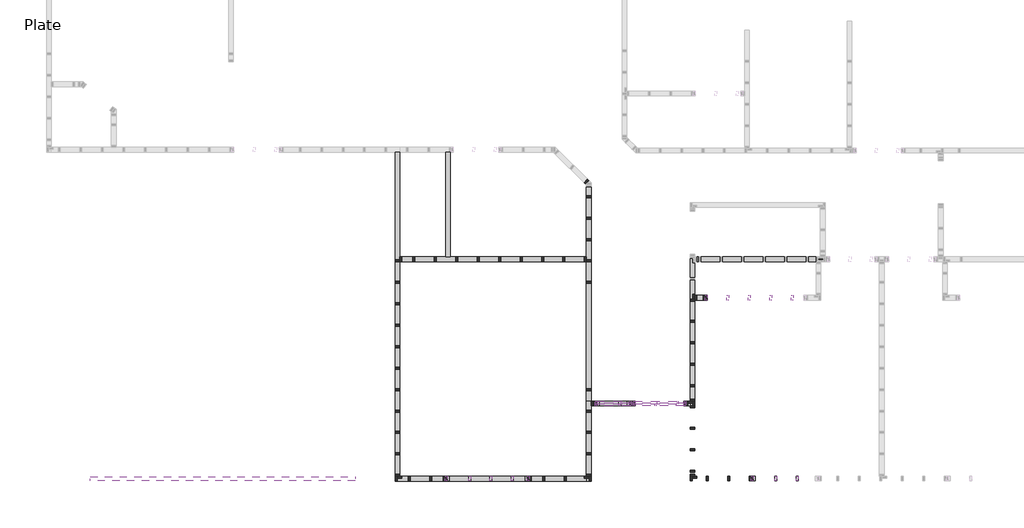
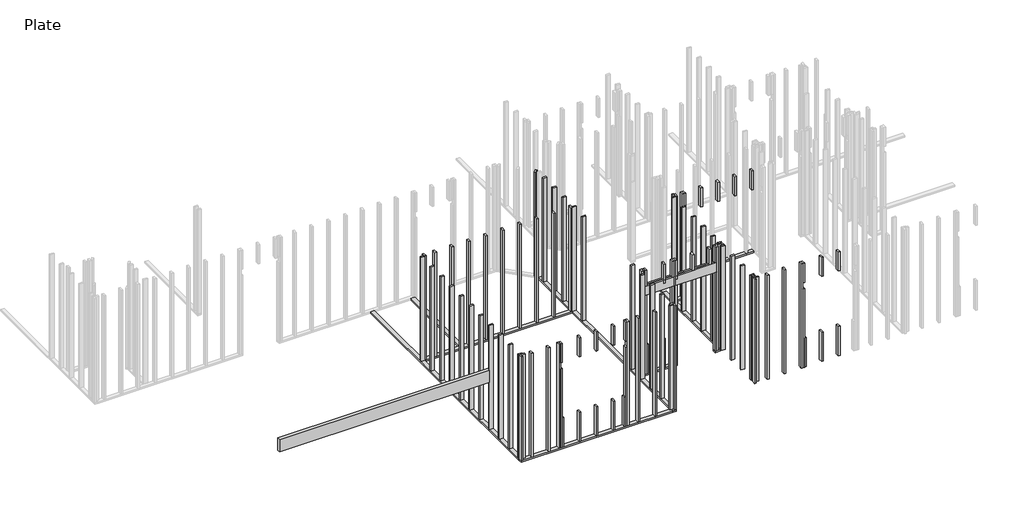
# One storey, part 1 of 5: 106 columns, 16 beams.
"""IFC4 building model written with IfcOpenShell, lengths in millimetres."""

import ifcopenshell
import ifcopenshell.guid

model = None  # the IFC model being written
_history = None  # IfcOwnerHistory: only IFC2X3 demands one
_inside = {}  # id of a spatial element -> (the spatial element, [elements in it])
_under = {}  # id of a project, library or spatial element -> (it, [spatial elements below it])
_declared = {}  # id of a project -> (the project, [libraries it declares])
_typed = {}  # id of a type object -> (the type object, [elements of that type])
_made_of = {}  # id of a material, layer set ... -> (it, [elements and type objects made of it])


def new_model(schema):
    """Start an empty IFC model of exactly this schema.

    Asked for "IFC4X3", IfcOpenShell would pick the latest addendum, in which some entities
    have other attributes; the version numbers below select the first issue.
    IFC2X3 requires an IfcOwnerHistory on every rooted entity: one is made here for all.
    """
    global model, _history
    if schema == "IFC4X3":
        model = ifcopenshell.file(schema_version=(4, 3, 0, 0))
    else:
        model = ifcopenshell.file(schema=schema)
    _inside.clear()
    _under.clear()
    _declared.clear()
    _typed.clear()
    _made_of.clear()
    _history = None
    if model.schema == "IFC2X3":
        org = make("IfcOrganization", Name="unknown")
        user = make(
            "IfcPersonAndOrganization",
            ThePerson=make("IfcPerson", FamilyName="unknown"),
            TheOrganization=org,
        )
        app = make(
            "IfcApplication",
            ApplicationDeveloper=org,
            Version="unknown",
            ApplicationFullName="unknown",
            ApplicationIdentifier="unknown",
        )
        _history = make(
            "IfcOwnerHistory",
            OwningUser=user,
            OwningApplication=app,
            ChangeAction="ADDED",
            CreationDate=0,
        )
    return model


def make(cls, **values):
    """One entity of the class cls with the attributes given. An attribute that is None is left unset."""
    return model.create_entity(
        cls, **{name: value for name, value in values.items() if value is not None}
    )


def rooted(cls, **values):
    """An entity with a GlobalId (a new one), such as an element, a storey or a relation."""
    return make(cls, GlobalId=ifcopenshell.guid.new(), OwnerHistory=_history, **values)


def si_unit(unit_type, name, prefix=None):
    """IfcSIUnit, for example si_unit("LENGTHUNIT", "METRE", prefix="MILLI")."""
    return make("IfcSIUnit", UnitType=unit_type, Prefix=prefix, Name=name)


def assignment(units):
    """IfcUnitAssignment: the units of a project."""
    return None if units is None else make("IfcUnitAssignment", Units=units)


def point(xyz):
    """IfcCartesianPoint."""
    return None if xyz is None else make("IfcCartesianPoint", Coordinates=xyz)


def direction(xyz):
    """IfcDirection."""
    return None if xyz is None else make("IfcDirection", DirectionRatios=xyz)


def frame(location, z_axis=None, x_axis=None):
    """IfcAxis2Placement3D, a coordinate frame: its origin and axes. An axis left out is left unset."""
    return make(
        "IfcAxis2Placement3D",
        Location=point(location),
        Axis=direction(z_axis),
        RefDirection=direction(x_axis),
    )


def origin():
    """The frame at (0, 0, 0) with its axes left unset."""
    return frame((0.0, 0.0, 0.0))


def place(relative_to, where):
    """IfcLocalPlacement: puts the frame where relative to a parent placement (None: the world)."""
    return make(
        "IfcLocalPlacement", PlacementRelTo=relative_to, RelativePlacement=where
    )


def context(
    kind, dimensions, precision=None, world=None, true_north=None, identifier=None
):
    """IfcGeometricRepresentationContext, for example the 3D "Model" context."""
    return make(
        "IfcGeometricRepresentationContext",
        ContextIdentifier=identifier,
        ContextType=kind,
        CoordinateSpaceDimension=dimensions,
        Precision=precision,
        WorldCoordinateSystem=world,
        TrueNorth=true_north,
    )


def project(units=None, contexts=None):
    """IfcProject with its units and contexts."""
    return rooted(
        "IfcProject",
        Name="project",
        RepresentationContexts=contexts,
        UnitsInContext=assignment(units),
    )


def spatial(cls, under=None, at=None, **own):
    """A site, building, storey or space (cls), placed at a placement, below another one or the project."""
    s = rooted(cls, ObjectPlacement=at, **own)
    if under is not None:
        _under.setdefault(under.id(), (under, []))[1].append(s)
    return s


def polyline(points):
    """IfcPolyline through the points."""
    return make("IfcPolyline", Points=[point(p) for p in points])


def outline(outer, holes=None, kind="AREA"):
    """IfcArbitraryClosedProfileDef: a profile drawn as a closed curve; with holes, ...WithVoids."""
    if holes is None:
        return make("IfcArbitraryClosedProfileDef", ProfileType=kind, OuterCurve=outer)
    return make(
        "IfcArbitraryProfileDefWithVoids",
        ProfileType=kind,
        OuterCurve=outer,
        InnerCurves=holes,
    )


def extrude(swept, where, along, depth):
    """IfcExtrudedAreaSolid: the profile swept, set in the frame where, extruded along a direction by depth."""
    return make(
        "IfcExtrudedAreaSolid",
        SweptArea=swept,
        Position=where,
        ExtrudedDirection=direction(along),
        Depth=depth,
    )


def shape(context_of_items, identifier, shape_type, items):
    """IfcShapeRepresentation: the items that make up one representation, for example the "Body"."""
    return make(
        "IfcShapeRepresentation",
        ContextOfItems=context_of_items,
        RepresentationIdentifier=identifier,
        RepresentationType=shape_type,
        Items=items,
    )


def source(mapping_origin, context_of_items, identifier, shape_type, items):
    """IfcRepresentationMap: a shape defined once, which mapped items show again and again."""
    return make(
        "IfcRepresentationMap",
        MappingOrigin=mapping_origin,
        MappedRepresentation=shape(context_of_items, identifier, shape_type, items),
    )


def transform(
    local_origin,
    x_axis=None,
    y_axis=None,
    z_axis=None,
    scale=None,
    scale2=None,
    scale3=None,
    uniform=True,
):
    """IfcCartesianTransformationOperator3D, or its non-uniform kind. x_axis, y_axis, z_axis: its Axis1, 2, 3."""
    if uniform:
        return make(
            "IfcCartesianTransformationOperator3D",
            Axis1=direction(x_axis),
            Axis2=direction(y_axis),
            LocalOrigin=point(local_origin),
            Scale=scale,
            Axis3=direction(z_axis),
        )
    return make(
        "IfcCartesianTransformationOperator3DnonUniform",
        Axis1=direction(x_axis),
        Axis2=direction(y_axis),
        LocalOrigin=point(local_origin),
        Scale=scale,
        Axis3=direction(z_axis),
        Scale2=scale2,
        Scale3=scale3,
    )


def mapped(mapping_source, mapping_target):
    """IfcMappedItem: shows the shape of a source again, moved by a transform."""
    return make(
        "IfcMappedItem", MappingSource=mapping_source, MappingTarget=mapping_target
    )


def made_of(thing, what):
    """Note that an element or type object is made of a material, layer set ...; save() writes the relation."""
    if what is not None:
        _made_of.setdefault(what.id(), (what, []))[1].append(thing)
    return thing


def element(
    cls,
    number,
    at=None,
    inside=None,
    cuts=None,
    type_object=None,
    material=None,
    context=None,
    identifier="Body",
    shape_type=None,
    held_by="IfcProductDefinitionShape",
    body=None,
    shapes=None,
    **own,
):
    """One element of the class cls, such as IfcWall. Its Tag is "e" and its number.

    at: its placement. inside: the storey or other place that contains it. cuts: it is an
    opening in that element (IfcRelVoidsElement). A single representation is given by context,
    identifier, shape_type and body (its items); several are given by shapes. held_by: the class
    of the entity that holds the representations. save() writes the other relations.
    """
    e = rooted(cls, Tag="e%d" % number, ObjectPlacement=at, **own)
    if body is not None:
        shapes = [shape(context, identifier, shape_type, body)]
    if shapes is not None:
        e.Representation = make(held_by, Representations=shapes)
    if inside is not None:
        _inside.setdefault(inside.id(), (inside, []))[1].append(e)
    if cuts is not None:
        rooted(
            "IfcRelVoidsElement", RelatingBuildingElement=cuts, RelatedOpeningElement=e
        )
    if type_object is not None:
        _typed.setdefault(type_object.id(), (type_object, []))[1].append(e)
    return made_of(e, material)


def aggregate(whole, parts):
    """IfcRelAggregates: a whole, such as a stair, and the parts it consists of."""
    return rooted("IfcRelAggregates", RelatingObject=whole, RelatedObjects=parts)


def save(model, path):
    """Write the relations noted so far, then the file.

    IfcRelAggregates (storeys below a building ...), IfcRelContainedInSpatialStructure (elements
    in a storey), IfcRelDefinesByType, IfcRelAssociatesMaterial and IfcRelDeclares: one each for
    every whole, place, type object, material and project.
    """
    for whole, parts in _under.values():
        aggregate(whole, parts)
    for where, things in _inside.values():
        rooted(
            "IfcRelContainedInSpatialStructure",
            RelatedElements=things,
            RelatingStructure=where,
        )
    for kind, things in _typed.values():
        rooted("IfcRelDefinesByType", RelatedObjects=things, RelatingType=kind)
    for what, things in _made_of.values():
        rooted("IfcRelAssociatesMaterial", RelatedObjects=things, RelatingMaterial=what)
    for by, libraries in _declared.values():
        rooted("IfcRelDeclares", RelatingContext=by, RelatedDefinitions=libraries)
    model.write(path)


def dimension_lumber_2x10_header_exterior_0c196d91(model_context):
    return source(origin(), model_context, "Body", "SweptSolid", [
        extrude(outline(polyline([(468.709375, 19.05), (468.709375, -19.05), (-217.090625, -19.05), (-217.090625, 19.05), (468.709375, 19.05)])), frame((0.0, 0.0, -117.475), z_axis=(0.0, 0.0, 1.0), x_axis=(1.0, 0.0, 0.0)), (0.0, 0.0, 1.0), 234.95),
    ])


def dimension_lumber_2x10_header_exterior_3e47137c(model_context):
    return source(origin(), model_context, "Body", "SweptSolid", [
        extrude(outline(polyline([(468.709375, 19.05), (468.709375, -19.05), (-521.890625, -19.05), (-521.890625, 19.05), (468.709375, 19.05)])), frame((0.0, 0.0, -117.475), z_axis=(0.0, 0.0, 1.0), x_axis=(1.0, 0.0, 0.0)), (0.0, 0.0, 1.0), 234.95),
    ])


def dimension_lumber_supporting_bottom_plate_a3b44643(model_context):
    return source(origin(), model_context, "Body", "SweptSolid", [
        extrude(outline(polyline([(84.225, 44.45), (84.225, -44.45), (-39.775, -44.45), (-39.775, 44.45), (84.225, 44.45)])), frame((0.0, 0.0, -19.05), z_axis=(0.0, 0.0, 1.0), x_axis=(1.0, 0.0, 0.0)), (0.0, 0.0, 1.0), 38.1),
    ])


def dimension_lumber_supporting_bottom_plate_5d1fa65a(model_context):
    return source(origin(), model_context, "Body", "SweptSolid", [
        extrude(outline(polyline([(755.65, 44.45), (755.65, -44.45), (-755.65, -44.45), (-755.65, 44.45), (755.65, 44.45)])), frame((0.0, 0.0, -19.05), z_axis=(0.0, 0.0, 1.0), x_axis=(1.0, 0.0, 0.0)), (0.0, 0.0, 1.0), 38.1),
    ])


def dimension_lumber_supporting_bottom_plate_2403c2db(model_context):
    return source(origin(), model_context, "Body", "SweptSolid", [
        extrude(outline(polyline([(1858.9625, 44.45), (1858.9625, -44.45), (-1770.0625, -44.45), (-1770.0625, 44.45), (1858.9625, 44.45)])), frame((0.0, 0.0, -19.05), z_axis=(0.0, 0.0, 1.0), x_axis=(1.0, 0.0, 0.0)), (0.0, 0.0, 1.0), 38.1),
    ])


def dimension_lumber_supporting_bottom_plate_8d258b52(model_context):
    return source(origin(), model_context, "Body", "SweptSolid", [
        extrude(outline(polyline([(3074.9875, 44.45), (3074.9875, -44.45), (-3074.9875, -44.45), (-3074.9875, 44.45), (3074.9875, 44.45)])), frame((0.0, 0.0, -19.05), z_axis=(0.0, 0.0, 1.0), x_axis=(1.0, 0.0, 0.0)), (0.0, 0.0, 1.0), 38.1),
    ])


def dimension_lumber_supporting_bottom_plate_bb9f9100(model_context):
    return source(origin(), model_context, "Body", "SweptSolid", [
        extrude(outline(polyline([(995.3625, 44.45), (995.3625, -44.45), (-995.3625, -44.45), (-995.3625, 44.45), (995.3625, 44.45)])), frame((0.0, 0.0, -19.05), z_axis=(0.0, 0.0, 1.0), x_axis=(1.0, 0.0, 0.0)), (0.0, 0.0, 1.0), 38.1),
    ])


def dimension_lumber_supporting_bottom_plate_9bff56d6(model_context):
    return source(origin(), model_context, "Body", "SweptSolid", [
        extrude(outline(polyline([(-1544.0421875, 44.45), (-1544.0421875, -44.45), (-4097.9328125, -44.45), (-4097.9328125, 44.45), (-1544.0421875, 44.45)])), frame((0.0, 0.0, -19.05), z_axis=(0.0, 0.0, 1.0), x_axis=(1.0, 0.0, 0.0)), (0.0, 0.0, 1.0), 38.1),
    ])


def dimension_lumber_supporting_bottom_plate_2ddee0ef(model_context):
    return source(origin(), model_context, "Body", "SweptSolid", [
        extrude(outline(polyline([(1771.65, 44.45), (1771.65, -44.45), (-1768.475, -44.45), (-1768.475, 44.45), (1771.65, 44.45)])), frame((0.0, 0.0, -19.05), z_axis=(0.0, 0.0, 1.0), x_axis=(1.0, 0.0, 0.0)), (0.0, 0.0, 1.0), 38.1),
    ])


def dimension_lumber_supporting_bottom_plate_736f332d(model_context):
    return source(origin(), model_context, "Body", "SweptSolid", [
        extrude(outline(polyline([(139.7000003, 44.45), (139.7000003, -44.45), (-95.2500003, -44.45), (-95.2500003, 44.45), (139.7000003, 44.45)])), frame((0.0, 0.0, -19.05), z_axis=(0.0, 0.0, 1.0), x_axis=(1.0, 0.0, 0.0)), (0.0, 0.0, 1.0), 38.1),
    ])


def dimension_lumber_supporting_bottom_plate_ae810c3f(model_context):
    return source(origin(), model_context, "Body", "SweptSolid", [
        extrude(outline(polyline([(1404.540625, 44.45), (1404.540625, -44.45), (-1385.490625, -44.45), (-1385.490625, 44.45), (1404.540625, 44.45)])), frame((0.0, 0.0, -19.05), z_axis=(0.0, 0.0, 1.0), x_axis=(1.0, 0.0, 0.0)), (0.0, 0.0, 1.0), 38.1),
    ])


def dimension_lumber_supporting_bottom_plate_d3939b75(model_context):
    return source(origin(), model_context, "Body", "SweptSolid", [
        extrude(outline(polyline([(398.375, 44.45), (398.375, -44.45), (-442.825, -44.45), (-442.825, 44.45), (398.375, 44.45)])), frame((0.0, 0.0, -19.05), z_axis=(0.0, 0.0, 1.0), x_axis=(1.0, 0.0, 0.0)), (0.0, 0.0, 1.0), 38.1),
    ])


def glulam_western_species_20871a06(model_context):
    return source(origin(), model_context, "Body", "SweptSolid", [
        extrude(outline(polyline([(481.409375, 39.6875), (481.409375, -39.6875), (-4547.790625, -39.6875), (-4547.790625, 39.6875), (481.409375, 39.6875)])), frame((0.0, 0.0, -152.4), z_axis=(0.0, 0.0, 1.0), x_axis=(1.0, 0.0, 0.0)), (0.0, 0.0, 1.0), 304.8),
    ])


def dimension_lumber_column_2x4_07183c39(model_context):
    return source(origin(), model_context, "Body", "SweptSolid", [
        extrude(outline(polyline([(19.05, 44.45), (19.05, -44.45), (-19.05, -44.45), (-19.05, 44.45), (19.05, 44.45)])), frame((0.0, 0.0, 56.35625), z_axis=(0.0, 0.0, 1.0), x_axis=(1.0, 0.0, 0.0)), (0.0, 0.0, 1.0), 2636.04375),
    ])


def dimension_lumber_column_2x4_f24b5bbb(model_context):
    return source(origin(), model_context, "Body", "SweptSolid", [
        extrude(outline(polyline([(19.05, -44.45), (-19.05, -44.45), (-19.05, 44.45), (19.05, 44.45), (19.05, -44.45)])), frame((0.0, 0.0, 56.35625), z_axis=(0.0, 0.0, 1.0), x_axis=(1.0, 0.0, 0.0)), (0.0, 0.0, 1.0), 2636.04375),
    ])


def dimension_lumber_column_2x4_0f816ddf(model_context):
    return source(origin(), model_context, "Body", "SweptSolid", [
        extrude(outline(polyline([(19.05, 44.45), (19.05, -44.45), (-19.05, -44.45), (-19.05, 44.45), (19.05, 44.45)])), frame((0.0, 0.0, 56.35625), z_axis=(0.0, 0.0, 1.0), x_axis=(1.0, 0.0, 0.0)), (0.0, 0.0, 1.0), 1999.853125),
    ])


def dimension_lumber_column_2x4_c2f848da(model_context):
    return source(origin(), model_context, "Body", "SweptSolid", [
        extrude(outline(polyline([(19.05, 44.45), (19.05, -44.45), (-19.05, -44.45), (-19.05, 44.45), (19.05, 44.45)])), frame((0.0, 0.0, 2208.609375), z_axis=(0.0, 0.0, 1.0), x_axis=(1.0, 0.0, 0.0)), (0.0, 0.0, 1.0), 483.790625),
    ])


def dimension_lumber_column_2x4_35883525(model_context):
    return source(origin(), model_context, "Body", "SweptSolid", [
        extrude(outline(polyline([(19.05, 44.45), (19.05, -44.45), (-19.05, -44.45), (-19.05, 44.45), (19.05, 44.45)])), frame((0.0, 0.0, 56.35625), z_axis=(0.0, 0.0, 1.0), x_axis=(1.0, 0.0, 0.0)), (0.0, 0.0, 1.0), 742.553125),
    ])


model = new_model("IFC4")

# Units and contexts
model_context = context("Model", 3, world=origin())
ifc_project = project(units=[si_unit("LENGTHUNIT", "METRE", prefix="MILLI")], contexts=[model_context])

# Site, building, storey
site = spatial("IfcSite", under=ifc_project)
building = spatial("IfcBuilding", under=site)
storey = spatial("IfcBuildingStorey", under=building, Name="Plate", Elevation=56.35625)

# Beams
placement = place(None, origin())
dimension_lumber_2x10_header_exterior_shape = dimension_lumber_2x10_header_exterior_0c196d91(model_context)
element("IfcBeam", 1, ObjectType="Dimension Lumber : 2x10 Header Exterior", at=placement, inside=storey, context=model_context, shape_type="MappedRepresentation", body=[
    mapped(dimension_lumber_2x10_header_exterior_shape, transform((4633.6941499, -4308.1040947, 2173.684375), x_axis=(-1.0, 0.0, 0.0), y_axis=(0.0, -1.0, 0.0), z_axis=(0.0, 0.0, 1.0))),
])
dimension_lumber_2x10_header_exterior_2_shape = dimension_lumber_2x10_header_exterior_3e47137c(model_context)
element("IfcBeam", 2, ObjectType="Dimension Lumber : 2x10 Header Exterior", at=placement, inside=storey, context=model_context, shape_type="MappedRepresentation", body=[
    mapped(dimension_lumber_2x10_header_exterior_2_shape, transform((5357.5941499, -4308.1040947, 2173.684375), x_axis=(-1.0, 0.0, 0.0), y_axis=(0.0, -1.0, 0.0), z_axis=(0.0, 0.0, 1.0))),
])
element("IfcBeam", 3, ObjectType="Dimension Lumber : 2x10 Header Interior", at=placement, inside=storey, context=model_context, shape_type="MappedRepresentation", body=[
    mapped(dimension_lumber_2x10_header_exterior_shape, transform((4633.6941499, -4257.3040947, 2173.684375), x_axis=(-1.0, 0.0, 0.0), y_axis=(0.0, -1.0, 0.0), z_axis=(0.0, 0.0, 1.0))),
])
element("IfcBeam", 4, ObjectType="Dimension Lumber : 2x10 Header Interior", at=placement, inside=storey, context=model_context, shape_type="MappedRepresentation", body=[
    mapped(dimension_lumber_2x10_header_exterior_2_shape, transform((5357.5941499, -4257.3040947, 2173.684375), x_axis=(-1.0, 0.0, 0.0), y_axis=(0.0, -1.0, 0.0), z_axis=(0.0, 0.0, 1.0))),
])
element("IfcBeam", 5, ObjectType="Dimension Lumber : Supporting Bottom Plate", at=placement, inside=storey, context=model_context, shape_type="SweptSolid", body=[
    extrude(outline(polyline([(4085.7847749, -4238.2540947), (3996.8847749, -4238.2540947), (3996.8847749, -134.8776804), (4085.7847749, -98.0540947), (4085.7847749, -4238.2540947)])), frame((0.0, 0.0, 18.25625), z_axis=(0.0, 0.0, 1.0), x_axis=(1.0, 0.0, 0.0)), (0.0, 0.0, 1.0), 38.1),
])
dimension_lumber_supporting_bottom_plate_shape = dimension_lumber_supporting_bottom_plate_a3b44643(model_context)
element("IfcBeam", 6, ObjectType="Dimension Lumber : Supporting Bottom Plate", at=placement, inside=storey, context=model_context, shape_type="MappedRepresentation", body=[
    mapped(dimension_lumber_supporting_bottom_plate_shape, transform((5925.6097749, -4282.7040947, 37.30625), x_axis=(-1.0, 0.0, 0.0), y_axis=(0.0, -1.0, 0.0), z_axis=(0.0, 0.0, 1.0))),
])
dimension_lumber_supporting_bottom_plate_2_shape = dimension_lumber_supporting_bottom_plate_5d1fa65a(model_context)
element("IfcBeam", 7, ObjectType="Dimension Lumber : Supporting Bottom Plate", at=placement, inside=storey, context=model_context, shape_type="MappedRepresentation", body=[
    mapped(dimension_lumber_supporting_bottom_plate_2_shape, transform((4041.3347749, -4993.9040947, 37.30625), x_axis=(0.0, -1.0, 0.0), y_axis=(1.0, 0.0, 0.0), z_axis=(0.0, 0.0, 1.0))),
])
dimension_lumber_supporting_bottom_plate_3_shape = dimension_lumber_supporting_bottom_plate_2403c2db(model_context)
element("IfcBeam", 8, ObjectType="Dimension Lumber : Supporting Bottom Plate", at=placement, inside=storey, context=model_context, shape_type="MappedRepresentation", body=[
    mapped(dimension_lumber_supporting_bottom_plate_3_shape, transform((2226.8222749, -5705.1040947, 37.30625), x_axis=(-1.0, 0.0, 0.0), y_axis=(0.0, -1.0, 0.0), z_axis=(0.0, 0.0, 1.0))),
])
dimension_lumber_supporting_bottom_plate_4_shape = dimension_lumber_supporting_bottom_plate_8d258b52(model_context)
element("IfcBeam", 9, ObjectType="Dimension Lumber : Supporting Bottom Plate", at=placement, inside=storey, context=model_context, shape_type="MappedRepresentation", body=[
    mapped(dimension_lumber_supporting_bottom_plate_4_shape, transform((412.3097749, -2585.6665947, 37.30625), x_axis=(0.0, 1.0, 0.0), y_axis=(-1.0, 0.0, 0.0), z_axis=(0.0, 0.0, 1.0))),
])
dimension_lumber_supporting_bottom_plate_5_shape = dimension_lumber_supporting_bottom_plate_bb9f9100(model_context)
element("IfcBeam", 10, ObjectType="Dimension Lumber : Supporting Bottom Plate", at=placement, inside=storey, context=model_context, shape_type="MappedRepresentation", body=[
    mapped(dimension_lumber_supporting_bottom_plate_5_shape, transform((1374.3347749, -506.0415947, 37.30625), x_axis=(0.0, -1.0, 0.0), y_axis=(1.0, 0.0, 0.0), z_axis=(0.0, 0.0, 1.0))),
])
dimension_lumber_supporting_bottom_plate_6_shape = dimension_lumber_supporting_bottom_plate_9bff56d6(model_context)
element("IfcBeam", 11, ObjectType="Dimension Lumber : Supporting Bottom Plate", at=placement, inside=storey, context=model_context, shape_type="MappedRepresentation", body=[
    mapped(dimension_lumber_supporting_bottom_plate_6_shape, transform((4510.2425874, -1545.8540947, 37.30625), x_axis=(-1.0, 0.0, 0.0), y_axis=(0.0, -1.0, 0.0), z_axis=(0.0, 0.0, 1.0))),
])
dimension_lumber_supporting_bottom_plate_7_shape = dimension_lumber_supporting_bottom_plate_2ddee0ef(model_context)
element("IfcBeam", 12, ObjectType="Dimension Lumber : Supporting Bottom Plate", at=placement, inside=storey, context=model_context, shape_type="MappedRepresentation", body=[
    mapped(dimension_lumber_supporting_bottom_plate_7_shape, transform((2225.2347749, -1545.8540947, 37.30625), x_axis=(1.0, 0.0, 0.0), y_axis=(0.0, 1.0, 0.0), z_axis=(0.0, 0.0, 1.0))),
])
dimension_lumber_supporting_bottom_plate_8_shape = dimension_lumber_supporting_bottom_plate_736f332d(model_context)
element("IfcBeam", 13, ObjectType="Dimension Lumber : Supporting Bottom Plate", at=placement, inside=storey, context=model_context, shape_type="MappedRepresentation", body=[
    mapped(dimension_lumber_supporting_bottom_plate_8_shape, transform((6149.5347752, -2276.1040947, 37.30625), x_axis=(1.0, 0.0, 0.0), y_axis=(0.0, 1.0, 0.0), z_axis=(0.0, 0.0, 1.0))),
])
dimension_lumber_supporting_bottom_plate_9_shape = dimension_lumber_supporting_bottom_plate_ae810c3f(model_context)
element("IfcBeam", 14, ObjectType="Dimension Lumber : Supporting Bottom Plate", at=placement, inside=storey, context=model_context, shape_type="MappedRepresentation", body=[
    mapped(dimension_lumber_supporting_bottom_plate_9_shape, transform((6009.8347749, -2833.7134697, 37.30625), x_axis=(0.0, -1.0, 0.0), y_axis=(1.0, 0.0, 0.0), z_axis=(0.0, 0.0, 1.0))),
])
dimension_lumber_supporting_bottom_plate_10_shape = dimension_lumber_supporting_bottom_plate_d3939b75(model_context)
element("IfcBeam", 15, ObjectType="Dimension Lumber : Supporting Bottom Plate", at=placement, inside=storey, context=model_context, shape_type="MappedRepresentation", body=[
    mapped(dimension_lumber_supporting_bottom_plate_10_shape, transform((4484.1597749, -4282.7040947, 37.30625), x_axis=(-1.0, 0.0, 0.0), y_axis=(0.0, -1.0, 0.0), z_axis=(0.0, 0.0, 1.0))),
])
glulam_western_species_shape = glulam_western_species_20871a06(model_context)
element("IfcBeam", 16, ObjectType="Glulam-Western Species : 3.125x12 Headers Exterior", at=placement, inside=storey, context=model_context, shape_type="MappedRepresentation", body=[
    mapped(glulam_western_species_shape, transform((-4932.4058501, -5705.1040947, 2457.45), x_axis=(-1.0, 0.0, 0.0), y_axis=(0.0, -1.0, 0.0), z_axis=(0.0, 0.0, 1.0))),
])

# Columns
dimension_lumber_column_2x4_shape = dimension_lumber_column_2x4_07183c39(model_context)
element("IfcColumn", 17, ObjectType="Dimension Lumber-Column : 2x4", at=placement, inside=storey, context=model_context, shape_type="MappedRepresentation", body=[
    mapped(dimension_lumber_column_2x4_shape, transform((6695.6347755, -5705.1040947, 0.0), x_axis=(1.0, 0.0, 0.0), y_axis=(0.0, 1.0, 0.0), z_axis=(0.0, 0.0, 1.0))),
])
element("IfcColumn", 18, ObjectType="Dimension Lumber-Column : 2x4", at=placement, inside=storey, context=model_context, shape_type="MappedRepresentation", body=[
    mapped(dimension_lumber_column_2x4_shape, transform((6289.2347755, -5705.1040947, 0.0), x_axis=(1.0, 0.0, 0.0), y_axis=(0.0, 1.0, 0.0), z_axis=(0.0, 0.0, 1.0))),
])
element("IfcColumn", 19, ObjectType="Dimension Lumber-Column : 2x4", at=placement, inside=storey, context=model_context, shape_type="MappedRepresentation", body=[
    mapped(dimension_lumber_column_2x4_shape, transform((5984.4347749, -5705.1040947, 0.0), x_axis=(1.0, 0.0, 0.0), y_axis=(0.0, 1.0, 0.0), z_axis=(0.0, 0.0, 1.0))),
])
element("IfcColumn", 20, ObjectType="Dimension Lumber-Column : 2x4", at=placement, inside=storey, context=model_context, shape_type="MappedRepresentation", body=[
    mapped(dimension_lumber_column_2x4_shape, transform((3596.8347749, -5705.1040947, 0.0), x_axis=(1.0, 0.0, 0.0), y_axis=(0.0, 1.0, 0.0), z_axis=(0.0, 0.0, 1.0))),
])
element("IfcColumn", 21, ObjectType="Dimension Lumber-Column : 2x4", at=placement, inside=storey, context=model_context, shape_type="MappedRepresentation", body=[
    mapped(dimension_lumber_column_2x4_shape, transform((3190.4347749, -5705.1040947, 0.0), x_axis=(1.0, 0.0, 0.0), y_axis=(0.0, 1.0, 0.0), z_axis=(0.0, 0.0, 1.0))),
])
element("IfcColumn", 22, ObjectType="Dimension Lumber-Column : 2x4", at=placement, inside=storey, context=model_context, shape_type="MappedRepresentation", body=[
    mapped(dimension_lumber_column_2x4_shape, transform((2936.4347749, -5705.1040947, 0.0), x_axis=(1.0, 0.0, 0.0), y_axis=(0.0, 1.0, 0.0), z_axis=(0.0, 0.0, 1.0))),
])
element("IfcColumn", 23, ObjectType="Dimension Lumber-Column : 2x4", at=placement, inside=storey, context=model_context, shape_type="MappedRepresentation", body=[
    mapped(dimension_lumber_column_2x4_shape, transform((1298.1347743, -5705.1040947, 0.0), x_axis=(1.0, 0.0, 0.0), y_axis=(0.0, 1.0, 0.0), z_axis=(0.0, 0.0, 1.0))),
])
element("IfcColumn", 24, ObjectType="Dimension Lumber-Column : 2x4", at=placement, inside=storey, context=model_context, shape_type="MappedRepresentation", body=[
    mapped(dimension_lumber_column_2x4_shape, transform((1044.1347749, -5705.1040947, 0.0), x_axis=(1.0, 0.0, 0.0), y_axis=(0.0, 1.0, 0.0), z_axis=(0.0, 0.0, 1.0))),
])
element("IfcColumn", 25, ObjectType="Dimension Lumber-Column : 2x4", at=placement, inside=storey, context=model_context, shape_type="MappedRepresentation", body=[
    mapped(dimension_lumber_column_2x4_shape, transform((637.7347749, -5705.1040947, 0.0), x_axis=(1.0, 0.0, 0.0), y_axis=(0.0, 1.0, 0.0), z_axis=(0.0, 0.0, 1.0))),
])
element("IfcColumn", 26, ObjectType="Dimension Lumber-Column : 2x4", at=placement, inside=storey, context=model_context, shape_type="MappedRepresentation", body=[
    mapped(dimension_lumber_column_2x4_shape, transform((4066.7347749, -5705.1040947, 0.0), x_axis=(1.0, 0.0, 0.0), y_axis=(0.0, 1.0, 0.0), z_axis=(0.0, 0.0, 1.0))),
])
element("IfcColumn", 27, ObjectType="Dimension Lumber-Column : 2x4", at=placement, inside=storey, context=model_context, shape_type="MappedRepresentation", body=[
    mapped(dimension_lumber_column_2x4_shape, transform((386.9097749, -5705.1040947, 0.0), x_axis=(1.0, 0.0, 0.0), y_axis=(0.0, 1.0, 0.0), z_axis=(0.0, 0.0, 1.0))),
])
element("IfcColumn", 28, ObjectType="Dimension Lumber-Column : 2x4", at=placement, inside=storey, context=model_context, shape_type="MappedRepresentation", body=[
    mapped(dimension_lumber_column_2x4_shape, transform((450.4097749, -5679.7040947, 0.0), x_axis=(0.0, 1.0, 0.0), y_axis=(-1.0, 0.0, 0.0), z_axis=(0.0, 0.0, 1.0))),
])
element("IfcColumn", 29, ObjectType="Dimension Lumber-Column : 2x4", at=placement, inside=storey, context=model_context, shape_type="MappedRepresentation", body=[
    mapped(dimension_lumber_column_2x4_shape, transform((7102.0347755, -5705.1040947, 0.0), x_axis=(1.0, 0.0, 0.0), y_axis=(0.0, 1.0, 0.0), z_axis=(0.0, 0.0, 1.0))),
])
element("IfcColumn", 30, ObjectType="Dimension Lumber-Column : 2x4", at=placement, inside=storey, context=model_context, shape_type="MappedRepresentation", body=[
    mapped(dimension_lumber_column_2x4_shape, transform((4104.8347749, -4282.7040947, 0.0), x_axis=(1.0, 0.0, 0.0), y_axis=(0.0, 1.0, 0.0), z_axis=(0.0, 0.0, 1.0))),
])
element("IfcColumn", 31, ObjectType="Dimension Lumber-Column : 2x4", at=placement, inside=storey, context=model_context, shape_type="MappedRepresentation", body=[
    mapped(dimension_lumber_column_2x4_shape, transform((6009.8347749, -4346.2040947, 0.0), x_axis=(0.0, 1.0, 0.0), y_axis=(-1.0, 0.0, 0.0), z_axis=(0.0, 0.0, 1.0))),
])
element("IfcColumn", 32, ObjectType="Dimension Lumber-Column : 2x4", at=placement, inside=storey, context=model_context, shape_type="MappedRepresentation", body=[
    mapped(dimension_lumber_column_2x4_shape, transform((5971.7347749, -4257.3040947, 0.0), x_axis=(0.0, 1.0, 0.0), y_axis=(-1.0, 0.0, 0.0), z_axis=(0.0, 0.0, 1.0))),
])
element("IfcColumn", 33, ObjectType="Dimension Lumber-Column : 2x4", at=placement, inside=storey, context=model_context, shape_type="MappedRepresentation", body=[
    mapped(dimension_lumber_column_2x4_shape, transform((6009.8347749, -4752.6040947, 0.0), x_axis=(0.0, 1.0, 0.0), y_axis=(-1.0, 0.0, 0.0), z_axis=(0.0, 0.0, 1.0))),
])
element("IfcColumn", 34, ObjectType="Dimension Lumber-Column : 2x4", at=placement, inside=storey, context=model_context, shape_type="MappedRepresentation", body=[
    mapped(dimension_lumber_column_2x4_shape, transform((6009.8347749, -5159.0040947, 0.0), x_axis=(0.0, 1.0, 0.0), y_axis=(-1.0, 0.0, 0.0), z_axis=(0.0, 0.0, 1.0))),
])
element("IfcColumn", 35, ObjectType="Dimension Lumber-Column : 2x4", at=placement, inside=storey, context=model_context, shape_type="MappedRepresentation", body=[
    mapped(dimension_lumber_column_2x4_shape, transform((6009.8347749, -5565.4040947, 0.0), x_axis=(0.0, 1.0, 0.0), y_axis=(-1.0, 0.0, 0.0), z_axis=(0.0, 0.0, 1.0))),
])
element("IfcColumn", 36, ObjectType="Dimension Lumber-Column : 2x4", at=placement, inside=storey, context=model_context, shape_type="MappedRepresentation", body=[
    mapped(dimension_lumber_column_2x4_shape, transform((6009.8347749, -5641.6040947, 0.0), x_axis=(0.0, 1.0, 0.0), y_axis=(-1.0, 0.0, 0.0), z_axis=(0.0, 0.0, 1.0))),
])
element("IfcColumn", 37, ObjectType="Dimension Lumber-Column : 2x4", at=placement, inside=storey, context=model_context, shape_type="MappedRepresentation", body=[
    mapped(dimension_lumber_column_2x4_shape, transform((6047.9347749, -5679.7040947, 0.0), x_axis=(0.0, 1.0, 0.0), y_axis=(-1.0, 0.0, 0.0), z_axis=(0.0, 0.0, 1.0))),
])
element("IfcColumn", 38, ObjectType="Dimension Lumber-Column : 2x4", at=placement, inside=storey, context=model_context, shape_type="MappedRepresentation", body=[
    mapped(dimension_lumber_column_2x4_shape, transform((3996.4334943, -71.5646069, 0.0), x_axis=(0.7071067811865461, -0.707106781186549, 0.0), y_axis=(0.707106781186549, 0.7071067811865461, 0.0), z_axis=(0.0, 0.0, 1.0))),
])
element("IfcColumn", 39, ObjectType="Dimension Lumber-Column : 2x4", at=placement, inside=storey, context=model_context, shape_type="MappedRepresentation", body=[
    mapped(dimension_lumber_column_2x4_shape, transform((3977.8347749, -1545.8540947, 0.0), x_axis=(1.0, 0.0, 0.0), y_axis=(0.0, 1.0, 0.0), z_axis=(0.0, 0.0, 1.0))),
])
element("IfcColumn", 40, ObjectType="Dimension Lumber-Column : 2x4", at=placement, inside=storey, context=model_context, shape_type="MappedRepresentation", body=[
    mapped(dimension_lumber_column_2x4_shape, transform((3571.4347749, -1545.8540947, 0.0), x_axis=(1.0, 0.0, 0.0), y_axis=(0.0, 1.0, 0.0), z_axis=(0.0, 0.0, 1.0))),
])
element("IfcColumn", 41, ObjectType="Dimension Lumber-Column : 2x4", at=placement, inside=storey, context=model_context, shape_type="MappedRepresentation", body=[
    mapped(dimension_lumber_column_2x4_shape, transform((3165.0347749, -1545.8540947, 0.0), x_axis=(1.0, 0.0, 0.0), y_axis=(0.0, 1.0, 0.0), z_axis=(0.0, 0.0, 1.0))),
])
element("IfcColumn", 42, ObjectType="Dimension Lumber-Column : 2x4", at=placement, inside=storey, context=model_context, shape_type="MappedRepresentation", body=[
    mapped(dimension_lumber_column_2x4_shape, transform((2758.6347749, -1545.8540947, 0.0), x_axis=(1.0, 0.0, 0.0), y_axis=(0.0, 1.0, 0.0), z_axis=(0.0, 0.0, 1.0))),
])
element("IfcColumn", 43, ObjectType="Dimension Lumber-Column : 2x4", at=placement, inside=storey, context=model_context, shape_type="MappedRepresentation", body=[
    mapped(dimension_lumber_column_2x4_shape, transform((2352.2347749, -1545.8540947, 0.0), x_axis=(1.0, 0.0, 0.0), y_axis=(0.0, 1.0, 0.0), z_axis=(0.0, 0.0, 1.0))),
])
element("IfcColumn", 44, ObjectType="Dimension Lumber-Column : 2x4", at=placement, inside=storey, context=model_context, shape_type="MappedRepresentation", body=[
    mapped(dimension_lumber_column_2x4_shape, transform((1945.8347749, -1545.8540947, 0.0), x_axis=(1.0, 0.0, 0.0), y_axis=(0.0, 1.0, 0.0), z_axis=(0.0, 0.0, 1.0))),
])
element("IfcColumn", 45, ObjectType="Dimension Lumber-Column : 2x4", at=placement, inside=storey, context=model_context, shape_type="MappedRepresentation", body=[
    mapped(dimension_lumber_column_2x4_shape, transform((1539.4347749, -1545.8540947, 0.0), x_axis=(1.0, 0.0, 0.0), y_axis=(0.0, 1.0, 0.0), z_axis=(0.0, 0.0, 1.0))),
])
element("IfcColumn", 46, ObjectType="Dimension Lumber-Column : 2x4", at=placement, inside=storey, context=model_context, shape_type="MappedRepresentation", body=[
    mapped(dimension_lumber_column_2x4_shape, transform((1133.0347749, -1545.8540947, 0.0), x_axis=(1.0, 0.0, 0.0), y_axis=(0.0, 1.0, 0.0), z_axis=(0.0, 0.0, 1.0))),
])
element("IfcColumn", 47, ObjectType="Dimension Lumber-Column : 2x4", at=placement, inside=storey, context=model_context, shape_type="MappedRepresentation", body=[
    mapped(dimension_lumber_column_2x4_shape, transform((726.6347749, -1545.8540947, 0.0), x_axis=(1.0, 0.0, 0.0), y_axis=(0.0, 1.0, 0.0), z_axis=(0.0, 0.0, 1.0))),
])
element("IfcColumn", 48, ObjectType="Dimension Lumber-Column : 2x4", at=placement, inside=storey, context=model_context, shape_type="MappedRepresentation", body=[
    mapped(dimension_lumber_column_2x4_shape, transform((475.8097749, -1545.8540947, 0.0), x_axis=(1.0, 0.0, 0.0), y_axis=(0.0, 1.0, 0.0), z_axis=(0.0, 0.0, 1.0))),
])
element("IfcColumn", 49, ObjectType="Dimension Lumber-Column : 2x4", at=placement, inside=storey, context=model_context, shape_type="MappedRepresentation", body=[
    mapped(dimension_lumber_column_2x4_shape, transform((4145.9347749, -4282.7040947, 0.0), x_axis=(1.0, 0.0, 0.0), y_axis=(0.0, 1.0, 0.0), z_axis=(0.0, 0.0, 1.0))),
])
element("IfcColumn", 50, ObjectType="Dimension Lumber-Column : 2x4", at=placement, inside=storey, context=model_context, shape_type="MappedRepresentation", body=[
    mapped(dimension_lumber_column_2x4_shape, transform((6073.3347749, -2276.1040947, 0.0), x_axis=(1.0, 0.0, 0.0), y_axis=(0.0, 1.0, 0.0), z_axis=(0.0, 0.0, 1.0))),
])
element("IfcColumn", 51, ObjectType="Dimension Lumber-Column : 2x4", at=placement, inside=storey, context=model_context, shape_type="MappedRepresentation", body=[
    mapped(dimension_lumber_column_2x4_shape, transform((6035.2347749, -2254.6728447, 0.0), x_axis=(1.0, 0.0, 0.0), y_axis=(0.0, 1.0, 0.0), z_axis=(0.0, 0.0, 1.0))),
])
element("IfcColumn", 52, ObjectType="Dimension Lumber-Column : 2x4", at=placement, inside=storey, context=model_context, shape_type="MappedRepresentation", body=[
    mapped(dimension_lumber_column_2x4_shape, transform((6232.0847755, -2276.1040947, 0.0), x_axis=(1.0, 0.0, 0.0), y_axis=(0.0, 1.0, 0.0), z_axis=(0.0, 0.0, 1.0))),
])
dimension_lumber_column_2x4_2_shape = dimension_lumber_column_2x4_f24b5bbb(model_context)
element("IfcColumn", 53, ObjectType="Dimension Lumber-Column : 2x4", at=placement, inside=storey, context=model_context, shape_type="MappedRepresentation", body=[
    mapped(dimension_lumber_column_2x4_2_shape, transform((4041.3347749, -5641.6040947, 0.0), x_axis=(0.0, 1.0, 0.0), y_axis=(-1.0, 0.0, 0.0), z_axis=(0.0, 0.0, 1.0))),
])
element("IfcColumn", 54, ObjectType="Dimension Lumber-Column : 2x4", at=placement, inside=storey, context=model_context, shape_type="MappedRepresentation", body=[
    mapped(dimension_lumber_column_2x4_2_shape, transform((4003.2347749, -5679.7040947, 0.0), x_axis=(0.0, 1.0, 0.0), y_axis=(-1.0, 0.0, 0.0), z_axis=(0.0, 0.0, 1.0))),
])
element("IfcColumn", 55, ObjectType="Dimension Lumber-Column : 2x4", at=placement, inside=storey, context=model_context, shape_type="MappedRepresentation", body=[
    mapped(dimension_lumber_column_2x4_2_shape, transform((4041.3347749, -5235.2040947, 0.0), x_axis=(0.0, 1.0, 0.0), y_axis=(-1.0, 0.0, 0.0), z_axis=(0.0, 0.0, 1.0))),
])
element("IfcColumn", 56, ObjectType="Dimension Lumber-Column : 2x4", at=placement, inside=storey, context=model_context, shape_type="MappedRepresentation", body=[
    mapped(dimension_lumber_column_2x4_2_shape, transform((4041.3347749, -4828.8040947, 0.0), x_axis=(0.0, 1.0, 0.0), y_axis=(-1.0, 0.0, 0.0), z_axis=(0.0, 0.0, 1.0))),
])
element("IfcColumn", 57, ObjectType="Dimension Lumber-Column : 2x4", at=placement, inside=storey, context=model_context, shape_type="MappedRepresentation", body=[
    mapped(dimension_lumber_column_2x4_2_shape, transform((4041.3347749, -4422.4040947, 0.0), x_axis=(0.0, 1.0, 0.0), y_axis=(-1.0, 0.0, 0.0), z_axis=(0.0, 0.0, 1.0))),
])
element("IfcColumn", 58, ObjectType="Dimension Lumber-Column : 2x4", at=placement, inside=storey, context=model_context, shape_type="MappedRepresentation", body=[
    mapped(dimension_lumber_column_2x4_2_shape, transform((4041.3347749, -4016.0040947, 0.0), x_axis=(0.0, 1.0, 0.0), y_axis=(-1.0, 0.0, 0.0), z_axis=(0.0, 0.0, 1.0))),
])
element("IfcColumn", 59, ObjectType="Dimension Lumber-Column : 2x4", at=placement, inside=storey, context=model_context, shape_type="MappedRepresentation", body=[
    mapped(dimension_lumber_column_2x4_2_shape, transform((4041.3347749, -1984.0040947, 0.0), x_axis=(0.0, 1.0, 0.0), y_axis=(-1.0, 0.0, 0.0), z_axis=(0.0, 0.0, 1.0))),
])
element("IfcColumn", 60, ObjectType="Dimension Lumber-Column : 2x4", at=placement, inside=storey, context=model_context, shape_type="MappedRepresentation", body=[
    mapped(dimension_lumber_column_2x4_2_shape, transform((4041.3347749, -1577.6040947, 0.0), x_axis=(0.0, 1.0, 0.0), y_axis=(-1.0, 0.0, 0.0), z_axis=(0.0, 0.0, 1.0))),
])
element("IfcColumn", 61, ObjectType="Dimension Lumber-Column : 2x4", at=placement, inside=storey, context=model_context, shape_type="MappedRepresentation", body=[
    mapped(dimension_lumber_column_2x4_2_shape, transform((4041.3347749, -1171.2040947, 0.0), x_axis=(0.0, 1.0, 0.0), y_axis=(-1.0, 0.0, 0.0), z_axis=(0.0, 0.0, 1.0))),
])
element("IfcColumn", 62, ObjectType="Dimension Lumber-Column : 2x4", at=placement, inside=storey, context=model_context, shape_type="MappedRepresentation", body=[
    mapped(dimension_lumber_column_2x4_2_shape, transform((4041.3347749, -764.8040947, 0.0), x_axis=(0.0, 1.0, 0.0), y_axis=(-1.0, 0.0, 0.0), z_axis=(0.0, 0.0, 1.0))),
])
element("IfcColumn", 63, ObjectType="Dimension Lumber-Column : 2x4", at=placement, inside=storey, context=model_context, shape_type="MappedRepresentation", body=[
    mapped(dimension_lumber_column_2x4_2_shape, transform((4041.3347749, -358.4040947, 0.0), x_axis=(0.0, 1.0, 0.0), y_axis=(-1.0, 0.0, 0.0), z_axis=(0.0, 0.0, 1.0))),
])
element("IfcColumn", 64, ObjectType="Dimension Lumber-Column : 2x4", at=placement, inside=storey, context=model_context, shape_type="MappedRepresentation", body=[
    mapped(dimension_lumber_column_2x4_2_shape, transform((412.3097749, -5641.6040947, 0.0), x_axis=(0.0, 1.0, 0.0), y_axis=(-1.0, 0.0, 0.0), z_axis=(0.0, 0.0, 1.0))),
])
element("IfcColumn", 65, ObjectType="Dimension Lumber-Column : 2x4", at=placement, inside=storey, context=model_context, shape_type="MappedRepresentation", body=[
    mapped(dimension_lumber_column_2x4_2_shape, transform((412.3097749, -5235.2040947, 0.0), x_axis=(0.0, 1.0, 0.0), y_axis=(-1.0, 0.0, 0.0), z_axis=(0.0, 0.0, 1.0))),
])
element("IfcColumn", 66, ObjectType="Dimension Lumber-Column : 2x4", at=placement, inside=storey, context=model_context, shape_type="MappedRepresentation", body=[
    mapped(dimension_lumber_column_2x4_2_shape, transform((412.3097749, -4828.8040947, 0.0), x_axis=(0.0, 1.0, 0.0), y_axis=(-1.0, 0.0, 0.0), z_axis=(0.0, 0.0, 1.0))),
])
element("IfcColumn", 67, ObjectType="Dimension Lumber-Column : 2x4", at=placement, inside=storey, context=model_context, shape_type="MappedRepresentation", body=[
    mapped(dimension_lumber_column_2x4_2_shape, transform((412.3097749, -4422.4040947, 0.0), x_axis=(0.0, 1.0, 0.0), y_axis=(-1.0, 0.0, 0.0), z_axis=(0.0, 0.0, 1.0))),
])
element("IfcColumn", 68, ObjectType="Dimension Lumber-Column : 2x4", at=placement, inside=storey, context=model_context, shape_type="MappedRepresentation", body=[
    mapped(dimension_lumber_column_2x4_2_shape, transform((412.3097749, -4016.0040947, 0.0), x_axis=(0.0, 1.0, 0.0), y_axis=(-1.0, 0.0, 0.0), z_axis=(0.0, 0.0, 1.0))),
])
element("IfcColumn", 69, ObjectType="Dimension Lumber-Column : 2x4", at=placement, inside=storey, context=model_context, shape_type="MappedRepresentation", body=[
    mapped(dimension_lumber_column_2x4_2_shape, transform((412.3097749, -3609.6040947, 0.0), x_axis=(0.0, 1.0, 0.0), y_axis=(-1.0, 0.0, 0.0), z_axis=(0.0, 0.0, 1.0))),
])
element("IfcColumn", 70, ObjectType="Dimension Lumber-Column : 2x4", at=placement, inside=storey, context=model_context, shape_type="MappedRepresentation", body=[
    mapped(dimension_lumber_column_2x4_2_shape, transform((412.3097749, -3203.2040947, 0.0), x_axis=(0.0, 1.0, 0.0), y_axis=(-1.0, 0.0, 0.0), z_axis=(0.0, 0.0, 1.0))),
])
element("IfcColumn", 71, ObjectType="Dimension Lumber-Column : 2x4", at=placement, inside=storey, context=model_context, shape_type="MappedRepresentation", body=[
    mapped(dimension_lumber_column_2x4_2_shape, transform((412.3097749, -2796.8040947, 0.0), x_axis=(0.0, 1.0, 0.0), y_axis=(-1.0, 0.0, 0.0), z_axis=(0.0, 0.0, 1.0))),
])
element("IfcColumn", 72, ObjectType="Dimension Lumber-Column : 2x4", at=placement, inside=storey, context=model_context, shape_type="MappedRepresentation", body=[
    mapped(dimension_lumber_column_2x4_2_shape, transform((412.3097749, -2390.4040947, 0.0), x_axis=(0.0, 1.0, 0.0), y_axis=(-1.0, 0.0, 0.0), z_axis=(0.0, 0.0, 1.0))),
])
element("IfcColumn", 73, ObjectType="Dimension Lumber-Column : 2x4", at=placement, inside=storey, context=model_context, shape_type="MappedRepresentation", body=[
    mapped(dimension_lumber_column_2x4_2_shape, transform((412.3097749, -1984.0040947, 0.0), x_axis=(0.0, 1.0, 0.0), y_axis=(-1.0, 0.0, 0.0), z_axis=(0.0, 0.0, 1.0))),
])
element("IfcColumn", 74, ObjectType="Dimension Lumber-Column : 2x4", at=placement, inside=storey, context=model_context, shape_type="MappedRepresentation", body=[
    mapped(dimension_lumber_column_2x4_2_shape, transform((412.3097749, -1577.6040947, 0.0), x_axis=(0.0, 1.0, 0.0), y_axis=(-1.0, 0.0, 0.0), z_axis=(0.0, 0.0, 1.0))),
])
element("IfcColumn", 75, ObjectType="Dimension Lumber-Column : 2x4", at=placement, inside=storey, context=model_context, shape_type="MappedRepresentation", body=[
    mapped(dimension_lumber_column_2x4_2_shape, transform((6009.8347749, -2318.1728447, 0.0), x_axis=(0.0, -1.0, 0.0), y_axis=(1.0, 0.0, 0.0), z_axis=(0.0, 0.0, 1.0))),
])
element("IfcColumn", 76, ObjectType="Dimension Lumber-Column : 2x4", at=placement, inside=storey, context=model_context, shape_type="MappedRepresentation", body=[
    mapped(dimension_lumber_column_2x4_2_shape, transform((6009.8347749, -2724.5728447, 0.0), x_axis=(0.0, -1.0, 0.0), y_axis=(1.0, 0.0, 0.0), z_axis=(0.0, 0.0, 1.0))),
])
element("IfcColumn", 77, ObjectType="Dimension Lumber-Column : 2x4", at=placement, inside=storey, context=model_context, shape_type="MappedRepresentation", body=[
    mapped(dimension_lumber_column_2x4_2_shape, transform((6009.8347749, -3130.9728447, 0.0), x_axis=(0.0, -1.0, 0.0), y_axis=(1.0, 0.0, 0.0), z_axis=(0.0, 0.0, 1.0))),
])
element("IfcColumn", 78, ObjectType="Dimension Lumber-Column : 2x4", at=placement, inside=storey, context=model_context, shape_type="MappedRepresentation", body=[
    mapped(dimension_lumber_column_2x4_2_shape, transform((6009.8347749, -3537.3728447, 0.0), x_axis=(0.0, -1.0, 0.0), y_axis=(1.0, 0.0, 0.0), z_axis=(0.0, 0.0, 1.0))),
])
element("IfcColumn", 79, ObjectType="Dimension Lumber-Column : 2x4", at=placement, inside=storey, context=model_context, shape_type="MappedRepresentation", body=[
    mapped(dimension_lumber_column_2x4_2_shape, transform((6009.8347749, -3943.7728447, 0.0), x_axis=(0.0, -1.0, 0.0), y_axis=(1.0, 0.0, 0.0), z_axis=(0.0, 0.0, 1.0))),
])
element("IfcColumn", 80, ObjectType="Dimension Lumber-Column : 2x4", at=placement, inside=storey, context=model_context, shape_type="MappedRepresentation", body=[
    mapped(dimension_lumber_column_2x4_2_shape, transform((6009.8347749, -4219.2040947, 0.0), x_axis=(0.0, -1.0, 0.0), y_axis=(1.0, 0.0, 0.0), z_axis=(0.0, 0.0, 1.0))),
])
dimension_lumber_column_2x4_3_shape = dimension_lumber_column_2x4_0f816ddf(model_context)
element("IfcColumn", 81, ObjectType="Dimension Lumber-Column : 2x4", at=placement, inside=storey, context=model_context, shape_type="MappedRepresentation", body=[
    mapped(dimension_lumber_column_2x4_3_shape, transform((7140.1347755, -5705.1040947, 0.0), x_axis=(1.0, 0.0, 0.0), y_axis=(0.0, 1.0, 0.0), z_axis=(0.0, 0.0, 1.0))),
])
element("IfcColumn", 82, ObjectType="Dimension Lumber-Column : 2x4", at=placement, inside=storey, context=model_context, shape_type="MappedRepresentation", body=[
    mapped(dimension_lumber_column_2x4_3_shape, transform((2898.3347749, -5705.1040947, 0.0), x_axis=(1.0, 0.0, 0.0), y_axis=(0.0, 1.0, 0.0), z_axis=(0.0, 0.0, 1.0))),
])
element("IfcColumn", 83, ObjectType="Dimension Lumber-Column : 2x4", at=placement, inside=storey, context=model_context, shape_type="MappedRepresentation", body=[
    mapped(dimension_lumber_column_2x4_3_shape, transform((1336.2347743, -5705.1040947, 0.0), x_axis=(1.0, 0.0, 0.0), y_axis=(0.0, 1.0, 0.0), z_axis=(0.0, 0.0, 1.0))),
])
element("IfcColumn", 84, ObjectType="Dimension Lumber-Column : 2x4", at=placement, inside=storey, context=model_context, shape_type="MappedRepresentation", body=[
    mapped(dimension_lumber_column_2x4_3_shape, transform((4831.7347749, -4282.7040947, 0.0), x_axis=(1.0, 0.0, 0.0), y_axis=(0.0, 1.0, 0.0), z_axis=(0.0, 0.0, 1.0))),
])
element("IfcColumn", 85, ObjectType="Dimension Lumber-Column : 2x4", at=placement, inside=storey, context=model_context, shape_type="MappedRepresentation", body=[
    mapped(dimension_lumber_column_2x4_3_shape, transform((4184.0347749, -4282.7040947, 0.0), x_axis=(1.0, 0.0, 0.0), y_axis=(0.0, 1.0, 0.0), z_axis=(0.0, 0.0, 1.0))),
])
element("IfcColumn", 86, ObjectType="Dimension Lumber-Column : 2x4", at=placement, inside=storey, context=model_context, shape_type="MappedRepresentation", body=[
    mapped(dimension_lumber_column_2x4_3_shape, transform((5860.4347749, -4282.7040947, 0.0), x_axis=(1.0, 0.0, 0.0), y_axis=(0.0, 1.0, 0.0), z_axis=(0.0, 0.0, 1.0))),
])
element("IfcColumn", 87, ObjectType="Dimension Lumber-Column : 2x4", at=placement, inside=storey, context=model_context, shape_type="MappedRepresentation", body=[
    mapped(dimension_lumber_column_2x4_3_shape, transform((4907.9347749, -4282.7040947, 0.0), x_axis=(1.0, 0.0, 0.0), y_axis=(0.0, 1.0, 0.0), z_axis=(0.0, 0.0, 1.0))),
])
element("IfcColumn", 88, ObjectType="Dimension Lumber-Column : 2x4", at=placement, inside=storey, context=model_context, shape_type="MappedRepresentation", body=[
    mapped(dimension_lumber_column_2x4_3_shape, transform((6270.1847755, -2276.1040947, 0.0), x_axis=(1.0, 0.0, 0.0), y_axis=(0.0, 1.0, 0.0), z_axis=(0.0, 0.0, 1.0))),
])
dimension_lumber_column_2x4_4_shape = dimension_lumber_column_2x4_c2f848da(model_context)
element("IfcColumn", 89, ObjectType="Dimension Lumber-Column : 2x4", at=placement, inside=storey, context=model_context, shape_type="MappedRepresentation", body=[
    mapped(dimension_lumber_column_2x4_4_shape, transform((7584.6347755, -5705.1040947, 0.0), x_axis=(1.0, 0.0, 0.0), y_axis=(0.0, 1.0, 0.0), z_axis=(0.0, 0.0, 1.0))),
])
element("IfcColumn", 90, ObjectType="Dimension Lumber-Column : 2x4", at=placement, inside=storey, context=model_context, shape_type="MappedRepresentation", body=[
    mapped(dimension_lumber_column_2x4_4_shape, transform((7140.1347755, -5705.1040947, 0.0), x_axis=(1.0, 0.0, 0.0), y_axis=(0.0, 1.0, 0.0), z_axis=(0.0, 0.0, 1.0))),
])
element("IfcColumn", 91, ObjectType="Dimension Lumber-Column : 2x4", at=placement, inside=storey, context=model_context, shape_type="MappedRepresentation", body=[
    mapped(dimension_lumber_column_2x4_4_shape, transform((7991.0347755, -5705.1040947, 0.0), x_axis=(1.0, 0.0, 0.0), y_axis=(0.0, 1.0, 0.0), z_axis=(0.0, 0.0, 1.0))),
])
element("IfcColumn", 92, ObjectType="Dimension Lumber-Column : 2x4", at=placement, inside=storey, context=model_context, shape_type="MappedRepresentation", body=[
    mapped(dimension_lumber_column_2x4_4_shape, transform((2898.3347749, -5705.1040947, 0.0), x_axis=(1.0, 0.0, 0.0), y_axis=(0.0, 1.0, 0.0), z_axis=(0.0, 0.0, 1.0))),
])
element("IfcColumn", 93, ObjectType="Dimension Lumber-Column : 2x4", at=placement, inside=storey, context=model_context, shape_type="MappedRepresentation", body=[
    mapped(dimension_lumber_column_2x4_4_shape, transform((1780.7347743, -5705.1040947, 0.0), x_axis=(1.0, 0.0, 0.0), y_axis=(0.0, 1.0, 0.0), z_axis=(0.0, 0.0, 1.0))),
])
element("IfcColumn", 94, ObjectType="Dimension Lumber-Column : 2x4", at=placement, inside=storey, context=model_context, shape_type="MappedRepresentation", body=[
    mapped(dimension_lumber_column_2x4_4_shape, transform((1336.2347743, -5705.1040947, 0.0), x_axis=(1.0, 0.0, 0.0), y_axis=(0.0, 1.0, 0.0), z_axis=(0.0, 0.0, 1.0))),
])
element("IfcColumn", 95, ObjectType="Dimension Lumber-Column : 2x4", at=placement, inside=storey, context=model_context, shape_type="MappedRepresentation", body=[
    mapped(dimension_lumber_column_2x4_4_shape, transform((2187.1347743, -5705.1040947, 0.0), x_axis=(1.0, 0.0, 0.0), y_axis=(0.0, 1.0, 0.0), z_axis=(0.0, 0.0, 1.0))),
])
element("IfcColumn", 96, ObjectType="Dimension Lumber-Column : 2x4", at=placement, inside=storey, context=model_context, shape_type="MappedRepresentation", body=[
    mapped(dimension_lumber_column_2x4_4_shape, transform((4628.5347749, -4282.7040947, 0.0), x_axis=(1.0, 0.0, 0.0), y_axis=(0.0, 1.0, 0.0), z_axis=(0.0, 0.0, 1.0))),
])
element("IfcColumn", 97, ObjectType="Dimension Lumber-Column : 2x4", at=placement, inside=storey, context=model_context, shape_type="MappedRepresentation", body=[
    mapped(dimension_lumber_column_2x4_4_shape, transform((4184.0347749, -4282.7040947, 0.0), x_axis=(1.0, 0.0, 0.0), y_axis=(0.0, 1.0, 0.0), z_axis=(0.0, 0.0, 1.0))),
])
element("IfcColumn", 98, ObjectType="Dimension Lumber-Column : 2x4", at=placement, inside=storey, context=model_context, shape_type="MappedRepresentation", body=[
    mapped(dimension_lumber_column_2x4_4_shape, transform((2593.5347743, -5705.1040947, 0.0), x_axis=(1.0, 0.0, 0.0), y_axis=(0.0, 1.0, 0.0), z_axis=(0.0, 0.0, 1.0))),
])
element("IfcColumn", 99, ObjectType="Dimension Lumber-Column : 2x4", at=placement, inside=storey, context=model_context, shape_type="MappedRepresentation", body=[
    mapped(dimension_lumber_column_2x4_4_shape, transform((4831.7347749, -4282.7040947, 0.0), x_axis=(1.0, 0.0, 0.0), y_axis=(0.0, 1.0, 0.0), z_axis=(0.0, 0.0, 1.0))),
])
element("IfcColumn", 100, ObjectType="Dimension Lumber-Column : 2x4", at=placement, inside=storey, context=model_context, shape_type="MappedRepresentation", body=[
    mapped(dimension_lumber_column_2x4_4_shape, transform((4907.9347749, -4282.7040947, 0.0), x_axis=(1.0, 0.0, 0.0), y_axis=(0.0, 1.0, 0.0), z_axis=(0.0, 0.0, 1.0))),
])
element("IfcColumn", 101, ObjectType="Dimension Lumber-Column : 2x4", at=placement, inside=storey, context=model_context, shape_type="MappedRepresentation", body=[
    mapped(dimension_lumber_column_2x4_4_shape, transform((5314.3347749, -4282.7040947, 0.0), x_axis=(1.0, 0.0, 0.0), y_axis=(0.0, 1.0, 0.0), z_axis=(0.0, 0.0, 1.0))),
])
element("IfcColumn", 102, ObjectType="Dimension Lumber-Column : 2x4", at=placement, inside=storey, context=model_context, shape_type="MappedRepresentation", body=[
    mapped(dimension_lumber_column_2x4_4_shape, transform((5720.7347749, -4282.7040947, 0.0), x_axis=(1.0, 0.0, 0.0), y_axis=(0.0, 1.0, 0.0), z_axis=(0.0, 0.0, 1.0))),
])
element("IfcColumn", 103, ObjectType="Dimension Lumber-Column : 2x4", at=placement, inside=storey, context=model_context, shape_type="MappedRepresentation", body=[
    mapped(dimension_lumber_column_2x4_4_shape, transform((5860.4347749, -4282.7040947, 0.0), x_axis=(1.0, 0.0, 0.0), y_axis=(0.0, 1.0, 0.0), z_axis=(0.0, 0.0, 1.0))),
])
element("IfcColumn", 104, ObjectType="Dimension Lumber-Column : 2x4", at=placement, inside=storey, context=model_context, shape_type="MappedRepresentation", body=[
    mapped(dimension_lumber_column_2x4_4_shape, transform((6270.1847755, -2276.1040947, 0.0), x_axis=(1.0, 0.0, 0.0), y_axis=(0.0, 1.0, 0.0), z_axis=(0.0, 0.0, 1.0))),
])
element("IfcColumn", 105, ObjectType="Dimension Lumber-Column : 2x4", at=placement, inside=storey, context=model_context, shape_type="MappedRepresentation", body=[
    mapped(dimension_lumber_column_2x4_4_shape, transform((6676.5847755, -2276.1040947, 0.0), x_axis=(1.0, 0.0, 0.0), y_axis=(0.0, 1.0, 0.0), z_axis=(0.0, 0.0, 1.0))),
])
element("IfcColumn", 106, ObjectType="Dimension Lumber-Column : 2x4", at=placement, inside=storey, context=model_context, shape_type="MappedRepresentation", body=[
    mapped(dimension_lumber_column_2x4_4_shape, transform((7082.9847755, -2276.1040947, 0.0), x_axis=(1.0, 0.0, 0.0), y_axis=(0.0, 1.0, 0.0), z_axis=(0.0, 0.0, 1.0))),
])
element("IfcColumn", 107, ObjectType="Dimension Lumber-Column : 2x4", at=placement, inside=storey, context=model_context, shape_type="MappedRepresentation", body=[
    mapped(dimension_lumber_column_2x4_4_shape, transform((7489.3847755, -2276.1040947, 0.0), x_axis=(1.0, 0.0, 0.0), y_axis=(0.0, 1.0, 0.0), z_axis=(0.0, 0.0, 1.0))),
])
element("IfcColumn", 108, ObjectType="Dimension Lumber-Column : 2x4", at=placement, inside=storey, context=model_context, shape_type="MappedRepresentation", body=[
    mapped(dimension_lumber_column_2x4_4_shape, transform((7895.7847755, -2276.1040947, 0.0), x_axis=(1.0, 0.0, 0.0), y_axis=(0.0, 1.0, 0.0), z_axis=(0.0, 0.0, 1.0))),
])
dimension_lumber_column_2x4_5_shape = dimension_lumber_column_2x4_35883525(model_context)
element("IfcColumn", 109, ObjectType="Dimension Lumber-Column : 2x4", at=placement, inside=storey, context=model_context, shape_type="MappedRepresentation", body=[
    mapped(dimension_lumber_column_2x4_5_shape, transform((7991.0347755, -5705.1040947, 0.0), x_axis=(1.0, 0.0, 0.0), y_axis=(0.0, 1.0, 0.0), z_axis=(0.0, 0.0, 1.0))),
])
element("IfcColumn", 110, ObjectType="Dimension Lumber-Column : 2x4", at=placement, inside=storey, context=model_context, shape_type="MappedRepresentation", body=[
    mapped(dimension_lumber_column_2x4_5_shape, transform((7584.6347755, -5705.1040947, 0.0), x_axis=(1.0, 0.0, 0.0), y_axis=(0.0, 1.0, 0.0), z_axis=(0.0, 0.0, 1.0))),
])
element("IfcColumn", 111, ObjectType="Dimension Lumber-Column : 2x4", at=placement, inside=storey, context=model_context, shape_type="MappedRepresentation", body=[
    mapped(dimension_lumber_column_2x4_5_shape, transform((7178.2347755, -5705.1040947, 0.0), x_axis=(1.0, 0.0, 0.0), y_axis=(0.0, 1.0, 0.0), z_axis=(0.0, 0.0, 1.0))),
])
element("IfcColumn", 112, ObjectType="Dimension Lumber-Column : 2x4", at=placement, inside=storey, context=model_context, shape_type="MappedRepresentation", body=[
    mapped(dimension_lumber_column_2x4_5_shape, transform((2187.1347743, -5705.1040947, 0.0), x_axis=(1.0, 0.0, 0.0), y_axis=(0.0, 1.0, 0.0), z_axis=(0.0, 0.0, 1.0))),
])
element("IfcColumn", 113, ObjectType="Dimension Lumber-Column : 2x4", at=placement, inside=storey, context=model_context, shape_type="MappedRepresentation", body=[
    mapped(dimension_lumber_column_2x4_5_shape, transform((1780.7347743, -5705.1040947, 0.0), x_axis=(1.0, 0.0, 0.0), y_axis=(0.0, 1.0, 0.0), z_axis=(0.0, 0.0, 1.0))),
])
element("IfcColumn", 114, ObjectType="Dimension Lumber-Column : 2x4", at=placement, inside=storey, context=model_context, shape_type="MappedRepresentation", body=[
    mapped(dimension_lumber_column_2x4_5_shape, transform((1374.3347743, -5705.1040947, 0.0), x_axis=(1.0, 0.0, 0.0), y_axis=(0.0, 1.0, 0.0), z_axis=(0.0, 0.0, 1.0))),
])
element("IfcColumn", 115, ObjectType="Dimension Lumber-Column : 2x4", at=placement, inside=storey, context=model_context, shape_type="MappedRepresentation", body=[
    mapped(dimension_lumber_column_2x4_5_shape, transform((2860.2347749, -5705.1040947, 0.0), x_axis=(1.0, 0.0, 0.0), y_axis=(0.0, 1.0, 0.0), z_axis=(0.0, 0.0, 1.0))),
])
element("IfcColumn", 116, ObjectType="Dimension Lumber-Column : 2x4", at=placement, inside=storey, context=model_context, shape_type="MappedRepresentation", body=[
    mapped(dimension_lumber_column_2x4_5_shape, transform((4628.5347749, -4282.7040947, 0.0), x_axis=(1.0, 0.0, 0.0), y_axis=(0.0, 1.0, 0.0), z_axis=(0.0, 0.0, 1.0))),
])
element("IfcColumn", 117, ObjectType="Dimension Lumber-Column : 2x4", at=placement, inside=storey, context=model_context, shape_type="MappedRepresentation", body=[
    mapped(dimension_lumber_column_2x4_5_shape, transform((4222.1347749, -4282.7040947, 0.0), x_axis=(1.0, 0.0, 0.0), y_axis=(0.0, 1.0, 0.0), z_axis=(0.0, 0.0, 1.0))),
])
element("IfcColumn", 118, ObjectType="Dimension Lumber-Column : 2x4", at=placement, inside=storey, context=model_context, shape_type="MappedRepresentation", body=[
    mapped(dimension_lumber_column_2x4_5_shape, transform((2593.5347743, -5705.1040947, 0.0), x_axis=(1.0, 0.0, 0.0), y_axis=(0.0, 1.0, 0.0), z_axis=(0.0, 0.0, 1.0))),
])
element("IfcColumn", 119, ObjectType="Dimension Lumber-Column : 2x4", at=placement, inside=storey, context=model_context, shape_type="MappedRepresentation", body=[
    mapped(dimension_lumber_column_2x4_5_shape, transform((4793.6347749, -4282.7040947, 0.0), x_axis=(1.0, 0.0, 0.0), y_axis=(0.0, 1.0, 0.0), z_axis=(0.0, 0.0, 1.0))),
])
element("IfcColumn", 120, ObjectType="Dimension Lumber-Column : 2x4", at=placement, inside=storey, context=model_context, shape_type="MappedRepresentation", body=[
    mapped(dimension_lumber_column_2x4_shape, transform((5898.5347749, -4282.7040947, 0.0), x_axis=(1.0, 0.0, 0.0), y_axis=(0.0, 1.0, 0.0), z_axis=(0.0, 0.0, 1.0))),
])
element("IfcColumn", 121, ObjectType="Dimension Lumber-Column : 2x4", at=placement, inside=storey, context=model_context, shape_type="MappedRepresentation", body=[
    mapped(dimension_lumber_column_2x4_shape, transform((6035.2347749, -4282.7040947, 0.0), x_axis=(1.0, 0.0, 0.0), y_axis=(0.0, 1.0, 0.0), z_axis=(0.0, 0.0, 1.0))),
])
element("IfcColumn", 122, ObjectType="Dimension Lumber-Column : 2x4", at=placement, inside=storey, context=model_context, shape_type="MappedRepresentation", body=[
    mapped(dimension_lumber_column_2x4_shape, transform((4869.8347749, -4282.7040947, 0.0), x_axis=(1.0, 0.0, 0.0), y_axis=(0.0, 1.0, 0.0), z_axis=(0.0, 0.0, 1.0))),
])

save(model, "model.ifc")
